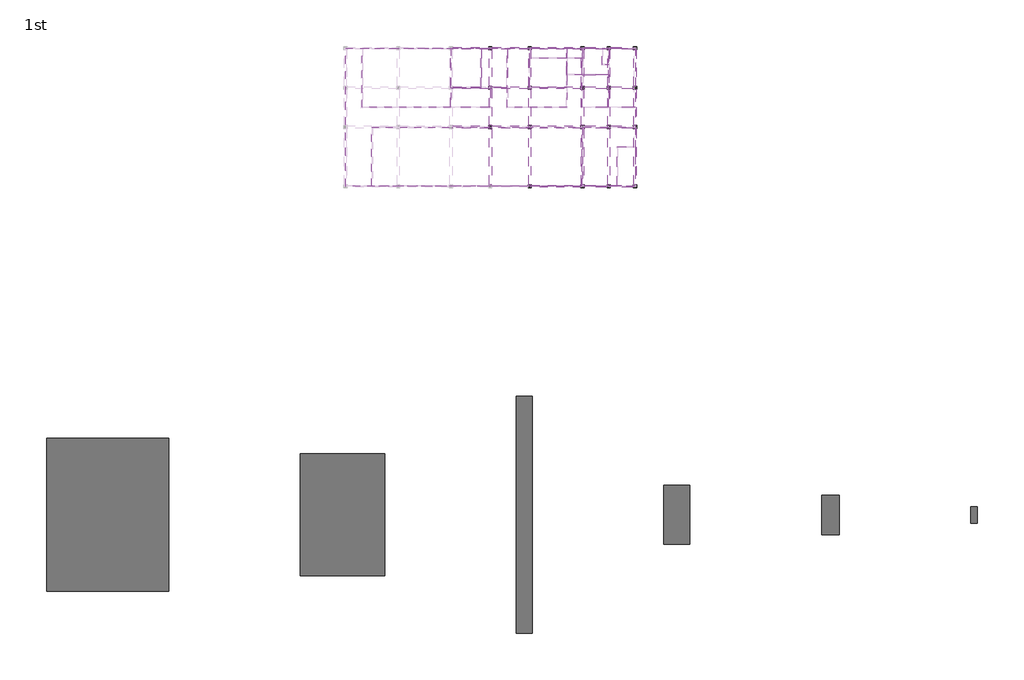
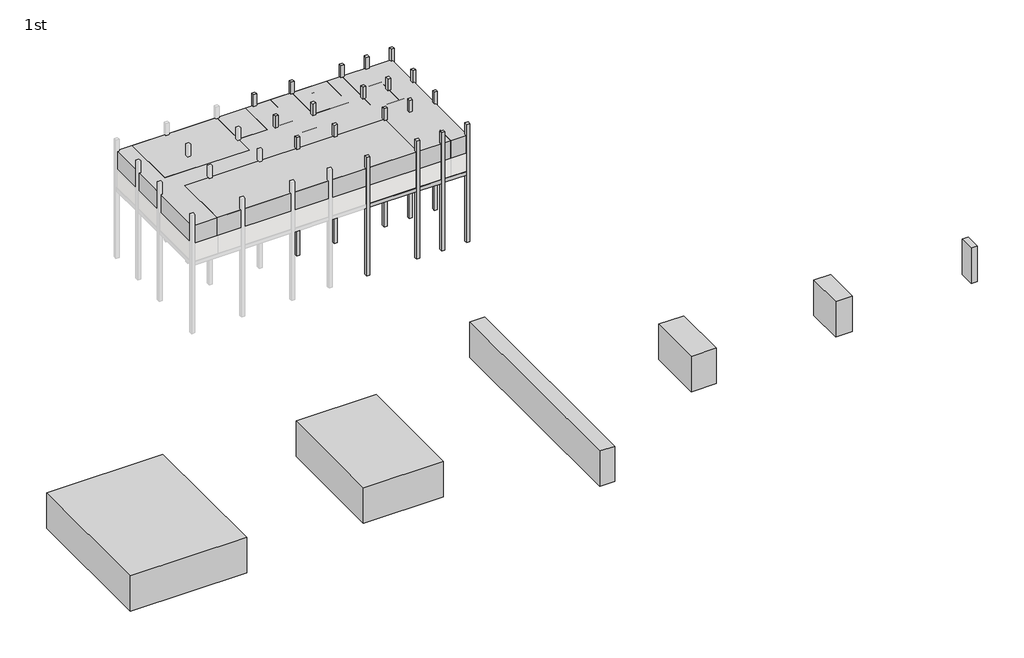
# One storey, part 3 of 3: 33 beams, 23 proxies, 19 columns.
# Revit data of these elements (continued)
# Element 54 (IfcBuildingElementProxy, "Space Planning Box_hec : Space Planning Box_hec") (continued)
#   Interior Finish = "IF2-1"
#   Exterior Finish = "EF1"
#   Department = "AR"
#   Width = 3000 mm
#   Program Area = 31.50 m²
#   Length = 6000 mm
#   Height = 6000 mm
#   Area = 18.00 m²
#   Fill Color = Lavender
#   Phase Created = New Construction
#   Materials on its faces: "Lavender"
# Element 55 (IfcBuildingElementProxy, "Space Planning Box_hec : Space Planning Box_hec")
#   Room Name = "Fire Gas Room"
#   Interior Finish = "IF1"
#   Exterior Finish = "EF1"
#   Department = "SF"
#   Width = 8000 mm
#   Program Area = 0.00 m²
#   Length = 9000 mm
#   Height = 6000 mm
#   Area = 72.00 m²
#   Fill Color = Cyan
#   Phase Created = New Construction
#   Materials on its faces: "Cyan"
# Element 56 (IfcBuildingElementProxy, "Space Planning Box_hec : Space Planning Box_hec")
#   Room Name = "Corridor"
#   Interior Finish = "IF2-1"
#   Exterior Finish = "EF1"
#   Department = "AR"
#   Width = 44000 mm
#   Program Area = 0.00 m²
#   Length = 21000 mm
#   Height = 6000 mm
#   Area = 924.00 m²
#   Fill Color = Lavender
#   Phase Created = New Construction
#   Materials on its faces: "Lavender"
# Elements 57, 58, 59, 60, 61, 62, 63, 64, 65, 66, 67, 68, 69, 70, 71, 72, 73, 74, 75 (IfcColumn, "Concrete-Rectangular-Column : CL111_500x500")
#   Comments = ""
#   hec_material3 = none
#   hec_material2 = none
#   hec_material1 = none
#   Structural Material = 콘크리트 - 현장타설 콘크리트
#   Phase Created = New Construction
#   Materials on its faces: "콘크리트 - 현장타설 콘크리트"
# Materials
#   "콘크리트 - 현장타설 콘크리트": class "콘크리트", colour RGB 192 192 192, transparency 0
#   "Cyan": class "Generic", colour RGB 0 255 255, transparency 0.2, Cost = 0
#   "A03AE056-00001_Bitumen/Bituminous/Asphalt Coating": class "Generic", colour RGB 17 17 17, transparency 0, Description = "Damp-proofing", W00) Work Master Code = "A03AE056-00001", W01) Work Master_Lv1 = "Concrete Work", W02) Work Master_Lv2 = "Concrete Protective Coating (U/G)", W03) Work Master_Spec.1 = "Bitumen/Bituminous/Asphalt Coating", Cost = 0
#   "A03AC035-00001_Form Work (3 times in use)_Flat": class "Wood", colour RGB 149 120 74, transparency 0, Description = "Plywood", W00) Work Master Code = "A03AC035-00001", W01) Work Master_Lv1 = "Concrete Work", W02) Work Master_Lv2 = "Substructure Work", W03) Work Master_Spec.1 = "Form Work (3 times in use)", W04) Work Master_Spec.2 = "Flat Form", W05) Work Master_Spec.3 = "Dressed Lumber, Plywood or Steel Form(Wood Planks are not Allowed) incl. Chamfer", Cost = 0
#   "A03AC032-00007_Structural Concrete_Type1_25MPa-30Mpa": class "Concrete", colour RGB 176 176 176, transparency 0, Keynote = "09910.A1", Description = "Reinf. Conc.", W00) Work Master Code = "A03AC032-00007", W01) Work Master_Lv1 = "Concrete Work", W02) Work Master_Lv2 = "Substructure Work", W03) Work Master_Spec.1 = "Structural Concrete", W04) Work Master_Spec.2 = "Cement Type-1", W05) Work Master_Spec.3 = "25MPa < F'c (Cylinder Strength) ≤ 30MPa", Cost = 0
#   "Lavender": class "Generic", colour RGB 186 85 211, transparency 0.2, Cost = 0
#   "Lime": class "Generic", colour RGB 0 255 0, transparency 0.2, Cost = 0
#   "Blue": class "Generic", colour RGB 0 0 255, transparency 0.2, Cost = 0
#   "Pink": class "Generic", colour RGB 255 105 180, transparency 0.2, Cost = 0
